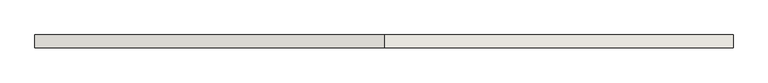
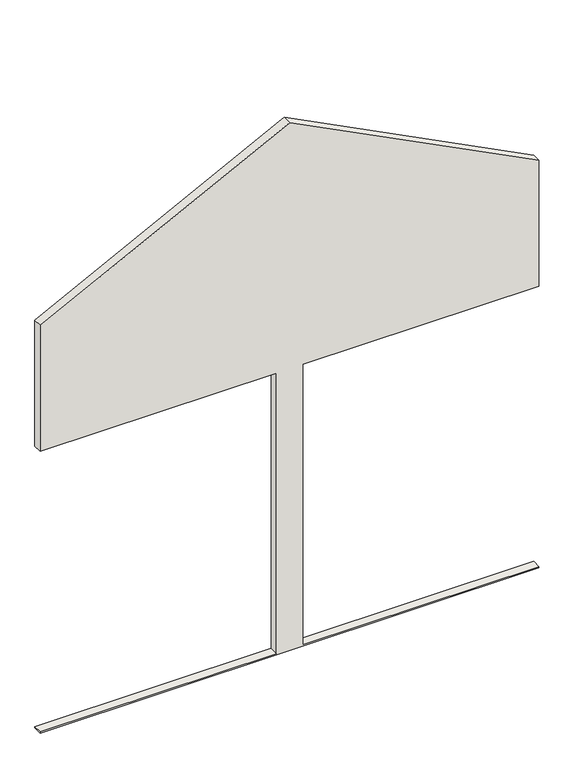
"""IFC4 building model written with IfcOpenShell, lengths in millimetres: wall geometry, 0_3d."""

from ifc_helpers import new_model, si_unit, frame, origin, place, context, project, spatial, polyline, outline, extrude, source, transform, mapped, element, save


def wall_46fbfe36(model_context):
    return source(origin(), model_context, "Body", "SweptSolid", [
        extrude(outline(polyline([(10.0, 3800.0), (10.0, 2000.0), (2270.0, 2000.0), (2270.0, 3800.0), (3283.5797924, 3800.0), (4251.6781465, 1900.0), (3283.5797924, 0.0), (2270.0, 0.0), (2270.0, 1800.0), (10.0, 1800.0), (10.0, 0.0), (0.0, 0.0), (0.0, 3800.0), (10.0, 3800.0)])), frame((0.0, 0.0, 0.0), z_axis=(0.0, 1.0, 0.0), x_axis=(0.0, 0.0, 1.0)), (0.0, 0.0, 1.0), 70.0),
    ])


if __name__ == "__main__":
    model = new_model("IFC4")
    model_context = context("Model", 3, world=origin())
    ifc_project = project(units=[si_unit("LENGTHUNIT", "METRE", prefix="MILLI")], contexts=[model_context])
    site = spatial("IfcSite", under=ifc_project)
    building = spatial("IfcBuilding", under=site)
    placement = place(None, origin())
    wall_shape = wall_46fbfe36(model_context)
    element("IfcWall", 1, ObjectType="0_3d", at=placement, inside=building, context=model_context, shape_type="MappedRepresentation", body=[
        mapped(wall_shape, transform((0.0, 0.0, 0.0), x_axis=(1.0, 0.0, 0.0), y_axis=(0.0, 1.0, 0.0), z_axis=(0.0, 0.0, 1.0))),
    ])
    save(model, "model.ifc")

# Revit data of these elements
# Element 1 (IfcWall, "0_3d")
#   Materials on its faces: "Glass_Simple"
# Materials
#   "Glass_Simple": class "Unassigned", colour RGB 255 255 255, transparency 0.9
